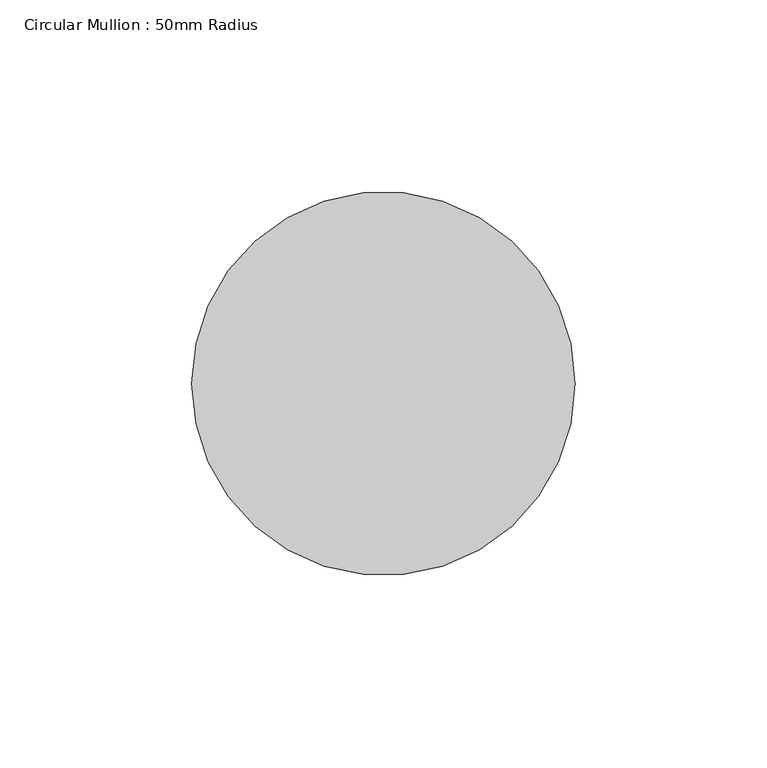
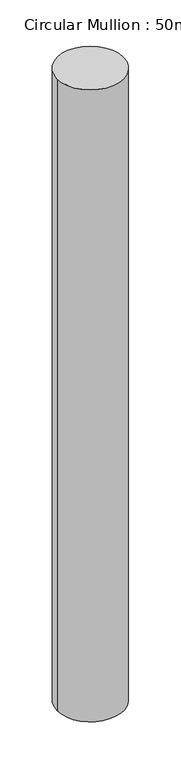
"""IFC4 building model written with IfcOpenShell, lengths in millimetres: member geometry, Circular Mullion : 50mm Radius."""

from ifc_helpers import new_model, si_unit, point, frame, origin, origin_2d, place, context, project, spatial, circle_curve, trimmed, segment, composite_curve, outline, extrude, source, transform, mapped, element, save


def circular_mullion_50mm_radius_89b22368(model_context):
    return source(origin(), model_context, "Body", "SweptSolid", [
        extrude(outline(composite_curve([segment(trimmed(circle_curve(origin_2d(), 50.0), [point((50.0, 0.0))], [point((-50.0, 0.0))], False, "CARTESIAN"), True, "CONTINUOUS"), segment(trimmed(circle_curve(origin_2d(), 50.0), [point((-50.0, 0.0))], [point((50.0, 0.0))], False, "CARTESIAN"), True, "CONTINUOUS")], self_intersect=False)), frame((0.0, 0.0, -1010.5477203), z_axis=(0.0, 0.0, 1.0), x_axis=(1.0, 0.0, 0.0)), (0.0, 0.0, 1.0), 1010.5477203),
    ])


if __name__ == "__main__":
    model = new_model("IFC4")
    model_context = context("Model", 3, world=origin())
    ifc_project = project(units=[si_unit("LENGTHUNIT", "METRE", prefix="MILLI")], contexts=[model_context])
    site = spatial("IfcSite", under=ifc_project)
    building = spatial("IfcBuilding", under=site)
    placement = place(None, origin())
    circular_mullion_50mm_radius_shape = circular_mullion_50mm_radius_89b22368(model_context)
    element("IfcMember", 1, ObjectType="Circular Mullion : 50mm Radius", at=placement, inside=building, context=model_context, shape_type="MappedRepresentation", body=[
        mapped(circular_mullion_50mm_radius_shape, transform((0.0, 0.0, 0.0), x_axis=(1.0, 0.0, 0.0), y_axis=(0.0, 1.0, 0.0), z_axis=(0.0, 0.0, 1.0))),
    ])
    save(model, "model.ifc")

# Revit data of these elements
# Type "Circular Mullion : 50mm Radius"
#   built-in parameter 1007350 = 0.164042 (stored number, unit not read)
# Element 1 (IfcMember, "Circular Mullion : 50mm Radius")
#   Materials on its faces: "Aluminium"
# Materials
#   "Aluminium": class "Metal", colour RGB 247 247 247, transparency 0, Description = "Aluminium 6061", Cost = 0
